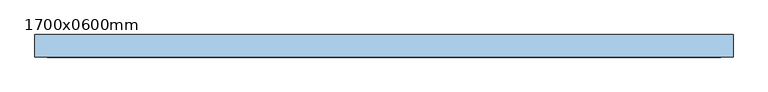
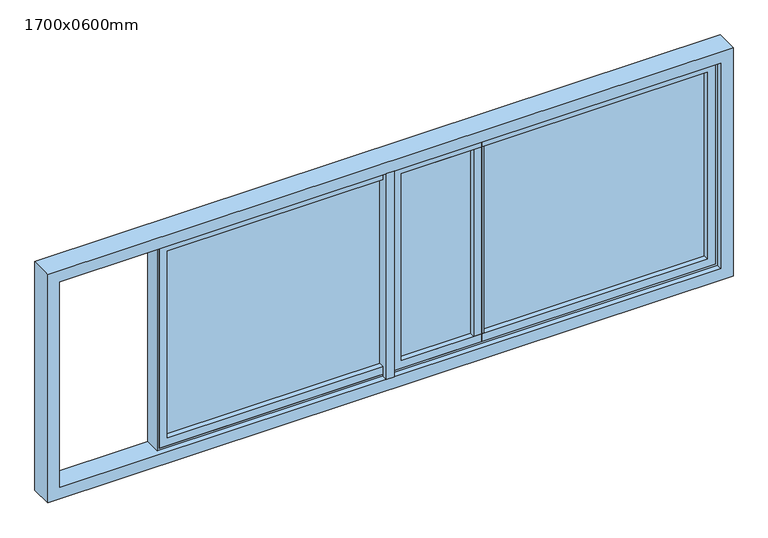
"""IFC4 building model written with IfcOpenShell, lengths in millimetres: window geometry, Janela Maxim-air - 2 Módulos : 1700x0600mm."""

from ifc_helpers import new_model, si_unit, frame, origin, place, context, project, spatial, polyline, outline, extrude, faceted_brep, source, transform, mapped, element, save


def window_1700x0600mm_ec30fa5b(model_context):
    return source(origin(), model_context, "Body", "SolidModel", [
        extrude(outline(polyline([(802.0, -51.3), (802.0, -58.3), (28.0, -58.3), (28.0, -51.3), (802.0, -51.3)])), frame((0.0, 0.0, 1048.0), z_axis=(0.0, 0.0, 1.0), x_axis=(1.0, 0.0, 0.0)), (0.0, 0.0, 1.0), 504.0),
        faceted_brep([(35.0, -72.3, 1545.0), (35.0, -72.3, 1055.0), (35.0, -58.3, 1055.0), (35.0, -58.3, 1545.0), (28.0, -58.3, 1552.0), (28.0, -58.3, 1048.0), (28.0, -51.3, 1048.0), (28.0, -51.3, 1552.0), (35.0, -51.3, 1545.0), (35.0, -51.3, 1055.0), (35.0, -37.3, 1055.0), (35.0, -37.3, 1545.0), (15.0, -37.3, 1565.0), (15.0, -37.3, 1035.0), (15.0, -72.3, 1035.0), (15.0, -72.3, 1565.0), (795.0, -72.3, 1055.0), (795.0, -58.3, 1055.0), (802.0, -58.3, 1048.0), (802.0, -51.3, 1048.0), (795.0, -51.3, 1055.0), (795.0, -37.3, 1055.0), (815.0, -37.3, 1035.0), (815.0, -72.3, 1035.0), (795.0, -72.3, 1545.0), (795.0, -58.3, 1545.0), (802.0, -58.3, 1552.0), (802.0, -51.3, 1552.0), (795.0, -51.3, 1545.0), (795.0, -37.3, 1545.0), (815.0, -37.3, 1565.0), (815.0, -72.3, 1565.0)], [[[0, 1, 2, 3]], [[4, 5, 6, 7]], [[8, 9, 10, 11]], [[12, 13, 14, 15]], [[1, 16, 17, 2]], [[5, 18, 19, 6]], [[9, 20, 21, 10]], [[13, 22, 23, 14]], [[16, 24, 25, 17]], [[18, 26, 27, 19]], [[20, 28, 29, 21]], [[22, 30, 31, 23]], [[15, 14, 23, 31], [1, 0, 24, 16]], [[24, 0, 3, 25]], [[5, 4, 26, 18], [3, 2, 17, 25]], [[26, 4, 7, 27]], [[7, 6, 19, 27], [9, 8, 28, 20]], [[28, 8, 11, 29]], [[13, 12, 30, 22], [11, 10, 21, 29]], [[30, 12, 15, 31]]]),
        faceted_brep([(15.0, -72.3, 1565.0), (15.0, -72.3, 1035.0), (15.0, -37.3, 1035.0), (15.0, -37.3, 1565.0), (20.0, -37.3, 1560.0), (20.0, -37.3, 1040.0), (20.0, -32.3, 1040.0), (20.0, -32.3, 1560.0), (10.0, -32.3, 1570.0), (10.0, -32.3, 1030.0), (10.0, -72.3, 1030.0), (10.0, -72.3, 1570.0), (815.0, -72.3, 1035.0), (815.0, -37.3, 1035.0), (810.0, -37.3, 1040.0), (810.0, -32.3, 1040.0), (820.0, -32.3, 1030.0), (820.0, -72.3, 1030.0), (815.0, -72.3, 1565.0), (815.0, -37.3, 1565.0), (810.0, -37.3, 1560.0), (810.0, -32.3, 1560.0), (820.0, -32.3, 1570.0), (820.0, -72.3, 1570.0)], [[[0, 1, 2, 3]], [[4, 5, 6, 7]], [[8, 9, 10, 11]], [[1, 12, 13, 2]], [[5, 14, 15, 6]], [[9, 16, 17, 10]], [[12, 18, 19, 13]], [[14, 20, 21, 15]], [[16, 22, 23, 17]], [[11, 10, 17, 23], [1, 0, 18, 12]], [[18, 0, 3, 19]], [[3, 2, 13, 19], [5, 4, 20, 14]], [[20, 4, 7, 21]], [[9, 8, 22, 16], [7, 6, 15, 21]], [[22, 8, 11, 23]]]),
        extrude(outline(polyline([(-552.0, -51.3), (222.0, -51.3), (222.0, -58.3), (-552.0, -58.3), (-552.0, -51.3)])), frame((0.0, 0.0, 1048.0), z_axis=(0.0, 0.0, 1.0), x_axis=(1.0, 0.0, 0.0)), (0.0, 0.0, 1.0), 504.0),
        faceted_brep([(215.0, -72.3, 1545.0), (215.0, -58.3, 1545.0), (215.0, -58.3, 1055.0), (215.0, -72.3, 1055.0), (222.0, -58.3, 1552.0), (222.0, -51.3, 1552.0), (222.0, -51.3, 1048.0), (222.0, -58.3, 1048.0), (215.0, -51.3, 1545.0), (215.0, -37.3, 1545.0), (215.0, -37.3, 1055.0), (215.0, -51.3, 1055.0), (235.0, -37.3, 1565.0), (235.0, -72.3, 1565.0), (235.0, -72.3, 1035.0), (235.0, -37.3, 1035.0), (-545.0, -58.3, 1055.0), (-545.0, -72.3, 1055.0), (-552.0, -51.3, 1048.0), (-552.0, -58.3, 1048.0), (-545.0, -37.3, 1055.0), (-545.0, -51.3, 1055.0), (-565.0, -72.3, 1035.0), (-565.0, -37.3, 1035.0), (-545.0, -58.3, 1545.0), (-545.0, -72.3, 1545.0), (-552.0, -51.3, 1552.0), (-552.0, -58.3, 1552.0), (-545.0, -37.3, 1545.0), (-545.0, -51.3, 1545.0), (-565.0, -72.3, 1565.0), (-565.0, -37.3, 1565.0)], [[[0, 1, 2, 3]], [[4, 5, 6, 7]], [[8, 9, 10, 11]], [[12, 13, 14, 15]], [[3, 2, 16, 17]], [[7, 6, 18, 19]], [[11, 10, 20, 21]], [[15, 14, 22, 23]], [[17, 16, 24, 25]], [[19, 18, 26, 27]], [[21, 20, 28, 29]], [[23, 22, 30, 31]], [[13, 30, 22, 14], [3, 17, 25, 0]], [[25, 24, 1, 0]], [[7, 19, 27, 4], [1, 24, 16, 2]], [[27, 26, 5, 4]], [[5, 26, 18, 6], [11, 21, 29, 8]], [[29, 28, 9, 8]], [[15, 23, 31, 12], [9, 28, 20, 10]], [[31, 30, 13, 12]]]),
        faceted_brep([(235.0, -72.3, 1565.0), (235.0, -37.3, 1565.0), (235.0, -37.3, 1035.0), (235.0, -72.3, 1035.0), (230.0, -37.3, 1560.0), (230.0, -32.3, 1560.0), (230.0, -32.3, 1040.0), (230.0, -37.3, 1040.0), (240.0, -32.3, 1570.0), (240.0, -72.3, 1570.0), (240.0, -72.3, 1030.0), (240.0, -32.3, 1030.0), (-565.0, -37.3, 1035.0), (-565.0, -72.3, 1035.0), (-560.0, -32.3, 1040.0), (-560.0, -37.3, 1040.0), (-570.0, -72.3, 1030.0), (-570.0, -32.3, 1030.0), (-565.0, -37.3, 1565.0), (-565.0, -72.3, 1565.0), (-560.0, -32.3, 1560.0), (-560.0, -37.3, 1560.0), (-570.0, -72.3, 1570.0), (-570.0, -32.3, 1570.0)], [[[0, 1, 2, 3]], [[4, 5, 6, 7]], [[8, 9, 10, 11]], [[3, 2, 12, 13]], [[7, 6, 14, 15]], [[11, 10, 16, 17]], [[13, 12, 18, 19]], [[15, 14, 20, 21]], [[17, 16, 22, 23]], [[9, 22, 16, 10], [3, 13, 19, 0]], [[19, 18, 1, 0]], [[1, 18, 12, 2], [7, 15, 21, 4]], [[21, 20, 5, 4]], [[11, 17, 23, 8], [5, 20, 14, 6]], [[23, 22, 9, 8]]]),
        extrude(outline(polyline([(10.0, -87.3), (-10.0, -87.3), (-10.0, -32.3), (10.0, -32.3), (10.0, -87.3)])), frame((0.0, 0.0, 1030.0), z_axis=(0.0, 0.0, 1.0), x_axis=(1.0, 0.0, 0.0)), (0.0, 0.0, 1.0), 540.0),
        extrude(outline(polyline([(1600.0, 850.0), (1600.0, -850.0), (1000.0, -850.0), (1000.0, 850.0), (1600.0, 850.0)]), holes=[polyline([(1030.0, 820.0), (1030.0, -820.0), (1570.0, -820.0), (1570.0, 820.0), (1030.0, 820.0)])]), frame((0.0, -87.3, 0.0), z_axis=(0.0, 1.0, 0.0), x_axis=(0.0, 0.0, 1.0)), (0.0, 0.0, 1.0), 55.0),
    ])


if __name__ == "__main__":
    model = new_model("IFC4")
    model_context = context("Model", 3, world=origin())
    ifc_project = project(units=[si_unit("LENGTHUNIT", "METRE", prefix="MILLI")], contexts=[model_context])
    site = spatial("IfcSite", under=ifc_project)
    building = spatial("IfcBuilding", under=site)
    placement = place(None, origin())
    window_1700x0600mm_shape = window_1700x0600mm_ec30fa5b(model_context)
    element("IfcWindow", 1, ObjectType="Janela Maxim-air - 2 Módulos : 1700x0600mm", at=placement, inside=building, context=model_context, shape_type="MappedRepresentation", body=[
        mapped(window_1700x0600mm_shape, transform((0.0, 0.0, 0.0), x_axis=(1.0, 0.0, 0.0), y_axis=(0.0, 1.0, 0.0), z_axis=(0.0, 0.0, 1.0))),
    ])
    save(model, "model.ifc")

# Revit data of these elements
# Type "Janela Maxim-air - 2 Módulos : 1700x0600mm"
#   Type Mark = "J2"
#   SINAPI = ""
#   ref. vert. basc. = 0.54 m
#   ref. horiz. basc. = 0.81 m
#   Largura Batente = 0.055 m
#   Height = 0.60 m
#   Default Sill Height = 1.00 m
#   Width = 1.70 m
#   Material Quadro = Metal - Alumínio
#   Material Painel = Vidro
#   Wall Closure = (empty or 0)
#   Assembly Code = ""
# Element 1 (IfcWindow, "Janela Maxim-air - 2 Módulos : 1700x0600mm")
#   Materials on its faces: "Metal - Alumínio", "Vidro"
# Materials
#   "Metal - Alumínio": class "Metal", colour RGB 244 244 244, transparency 0
#   "Vidro": class "Vidro", colour RGB 0 128 192, transparency 0.9, Description = "Vidro de sílica", Cost = 0
